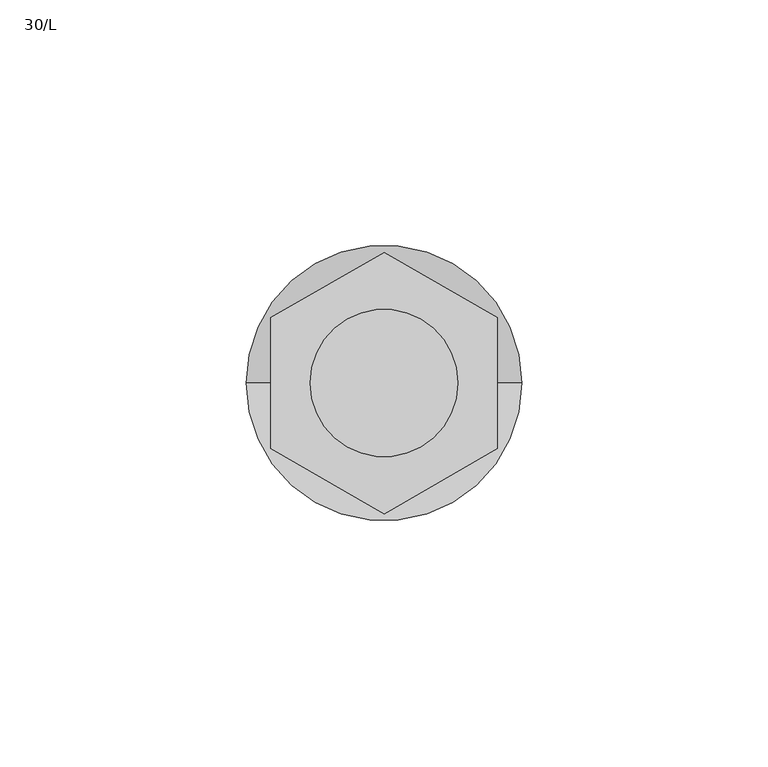
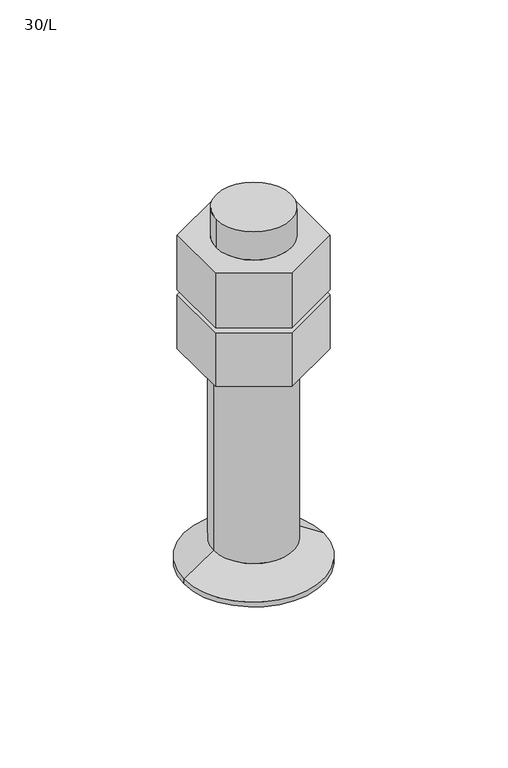
"""IFC4 building model written with IfcOpenShell, lengths in millimetres: fastener geometry, Bolt HPM-L : 30/L."""

from ifc_helpers import new_model, si_unit, frame, origin, origin_with_axes, place, context, project, spatial, polyline, circle_curve, source, transform, mapped, element, save
from ifc_brep_helpers import plane_surface, cylinder_surface, revolved_surface, advanced_brep


def fastener_30_l_a8502369(model_context):
    return source(origin(), model_context, "Body", "AdvancedBrep", [
        advanced_brep(
        [(-23.0, 13.2790562, 22.7), (-23.0, -13.2790562, 22.7), (0.0, -26.5581124, 22.7), (23.0, -13.2790562, 22.7), (23.0, 13.2790562, 22.7), (0.0, 26.5581124, 22.7), (15.0, 0.0, 22.7), (-15.0, 0.0, 22.7), (-23.0, 13.2790562, 0.0), (-23.0, -13.2790562, 0.0), (0.0, -26.5581124, 0.0), (23.0, -13.2790562, 0.0), (23.0, 13.2790562, 0.0), (0.0, 26.5581124, 0.0), (-15.0, 0.0, 60.0), (15.0, 0.0, 60.0), (15.0, 0.0, 25.0), (-15.0, 0.0, 25.0), (-15.0, 0.0, 48.0), (15.0, 0.0, 48.0), (-23.0, 13.2790562, 25.0), (0.0, 26.5581124, 25.0), (23.0, 13.2790562, 25.0), (23.0, -13.2790562, 25.0), (0.0, -26.5581124, 25.0), (-23.0, -13.2790562, 25.0), (-23.0, -13.2790562, 48.0), (-23.0, 13.2790562, 48.0), (0.0, -26.5581124, 48.0), (23.0, -13.2790562, 48.0), (23.0, 13.2790562, 48.0), (0.0, 26.5581124, 48.0), (-16.0, 0.0, 0.0), (-16.0, 0.0, -80.0), (16.0, 0.0, -80.0), (16.0, 0.0, 0.0), (-28.0, 0.0, -90.0), (28.0, 0.0, -90.0), (28.0, 0.0, -88.0), (-28.0, 0.0, -88.0)],
        [
            (0, 1),
            (1, 2),
            (2, 3),
            (3, 4),
            (4, 5),
            (5, 0),
            (6, 7, circle_curve(frame((0.0, 0.0, 22.7), z_axis=(0.0, 0.0, -1.0), x_axis=(1.0, 0.0, 0.0)), 15.0)),
            (7, 6, circle_curve(frame((0.0, 0.0, 22.7), z_axis=(0.0, 0.0, -1.0), x_axis=(1.0, 0.0, 0.0)), 15.0)),
            (0, 8),
            (8, 9),
            (9, 1),
            (9, 10),
            (10, 2),
            (10, 11),
            (11, 3),
            (11, 12),
            (12, 4),
            (12, 13),
            (13, 5),
            (13, 8),
            (14, 15, circle_curve(frame((0.0, 0.0, 60.0), z_axis=(0.0, 0.0, 1.0), x_axis=(1.0, 0.0, 0.0)), 15.0)),
            (15, 14, circle_curve(frame((0.0, 0.0, 60.0), z_axis=(0.0, 0.0, 1.0), x_axis=(1.0, 0.0, 0.0)), 15.0)),
            (6, 16),
            (16, 17, circle_curve(frame((0.0, 0.0, 25.0), z_axis=(0.0, 0.0, -1.0), x_axis=(1.0, 0.0, 0.0)), 15.0)),
            (17, 7),
            (14, 18),
            (18, 19, circle_curve(frame((0.0, 0.0, 48.0), z_axis=(0.0, 0.0, 1.0), x_axis=(1.0, 0.0, 0.0)), 15.0)),
            (19, 15),
            (17, 16, circle_curve(frame((0.0, 0.0, 25.0), z_axis=(0.0, 0.0, -1.0), x_axis=(1.0, 0.0, 0.0)), 15.0)),
            (19, 18, circle_curve(frame((0.0, 0.0, 48.0), z_axis=(0.0, 0.0, 1.0), x_axis=(1.0, 0.0, 0.0)), 15.0)),
            (20, 21),
            (21, 22),
            (22, 23),
            (23, 24),
            (24, 25),
            (25, 20),
            (26, 27),
            (27, 20),
            (25, 26),
            (28, 26),
            (24, 28),
            (29, 28),
            (23, 29),
            (30, 29),
            (22, 30),
            (31, 30),
            (21, 31),
            (27, 31),
            (32, 33),
            (33, 34, circle_curve(frame((0.0, 0.0, -80.0), z_axis=(0.0, 0.0, 1.0), x_axis=(1.0, 0.0, 0.0)), 16.0)),
            (34, 35),
            (35, 32, circle_curve(frame((0.0, 0.0, 0.0), z_axis=(0.0, 0.0, -1.0), x_axis=(1.0, 0.0, 0.0)), 16.0)),
            (32, 35, circle_curve(frame((0.0, 0.0, 0.0), z_axis=(0.0, 0.0, -1.0), x_axis=(1.0, 0.0, 0.0)), 16.0)),
            (34, 33, circle_curve(frame((0.0, 0.0, -80.0), z_axis=(0.0, 0.0, 1.0), x_axis=(1.0, 0.0, 0.0)), 16.0)),
            (36, 37, circle_curve(frame((0.0, 0.0, -90.0), z_axis=(0.0, 0.0, -1.0), x_axis=(1.0, 0.0, 0.0)), 28.0)),
            (37, 36, circle_curve(frame((0.0, 0.0, -90.0), z_axis=(0.0, 0.0, -1.0), x_axis=(1.0, 0.0, 0.0)), 28.0)),
            (37, 38),
            (38, 39, circle_curve(frame((0.0, 0.0, -88.0), z_axis=(0.0, 0.0, -1.0), x_axis=(1.0, 0.0, 0.0)), 28.0)),
            (39, 36),
            (39, 38, circle_curve(frame((0.0, 0.0, -88.0), z_axis=(0.0, 0.0, -1.0), x_axis=(1.0, 0.0, 0.0)), 28.0)),
            (33, 39),
            (38, 34),
        ],
        [
            plane_surface(frame((-23.0, 13.2790562, 22.7), z_axis=(0.0, 0.0, 1.0), x_axis=(0.0, -1.0, 0.0))),
            plane_surface(frame((-23.0, 13.2790562, 22.7), z_axis=(-1.0, 0.0, 0.0), x_axis=(0.0, 0.0, -1.0))),
            plane_surface(frame((-23.0, -13.2790562, 22.7), z_axis=(-0.4999999999999993, -0.8660254037844392, 0.0), x_axis=(0.0, 0.0, -1.0))),
            plane_surface(frame((0.0, -26.5581124, 22.7), z_axis=(0.5000000000000024, -0.8660254037844374, 0.0), x_axis=(0.0, 0.0, -1.0))),
            plane_surface(frame((23.0, -13.2790562, 22.7), z_axis=(1.0, 0.0, 0.0), x_axis=(0.0, 0.0, -1.0))),
            plane_surface(frame((23.0, 13.2790562, 22.7), z_axis=(0.4999999999999989, 0.8660254037844393, 0.0), x_axis=(0.0, 0.0, -1.0))),
            plane_surface(frame((0.0, 26.5581124, 22.7), z_axis=(-0.49999999999999895, 0.8660254037844393, 0.0), x_axis=(0.0, 0.0, -1.0))),
            plane_surface(frame((15.0, 0.0, 60.0), z_axis=(0.0, 0.0, 1.0), x_axis=(0.0, 1.0, 0.0))),
            cylinder_surface(origin_with_axes(), 15.0),
            plane_surface(frame((-23.0, 13.2790562, 25.0), z_axis=(0.0, 0.0, -1.0), x_axis=(0.0, 1.0, 0.0))),
            plane_surface(frame((-23.0, 13.2790562, 48.0), z_axis=(-1.0, 0.0, 0.0), x_axis=(0.0, 0.0, -1.0))),
            plane_surface(frame((-23.0, -13.2790562, 48.0), z_axis=(-0.4999999999999995, -0.866025403784439, 0.0), x_axis=(0.0, 0.0, -1.0))),
            plane_surface(frame((0.0, -26.5581124, 48.0), z_axis=(0.5000000000000024, -0.8660254037844373, 0.0), x_axis=(0.0, 0.0, -1.0))),
            plane_surface(frame((23.0, -13.2790562, 48.0), z_axis=(1.0, 0.0, 0.0), x_axis=(0.0, 0.0, -1.0))),
            plane_surface(frame((23.0, 13.2790562, 48.0), z_axis=(0.4999999999999991, 0.8660254037844393, 0.0), x_axis=(0.0, 0.0, -1.0))),
            plane_surface(frame((0.0, 26.5581124, 48.0), z_axis=(-0.49999999999999895, 0.8660254037844393, 0.0), x_axis=(0.0, 0.0, -1.0))),
            cylinder_surface(frame((0.0, 0.0, -80.0), z_axis=(0.0, 0.0, 1.0), x_axis=(1.0, 0.0, 0.0)), 16.0),
            plane_surface(frame((28.0, 0.0, -90.0), z_axis=(0.0, 0.0, -1.0), x_axis=(0.0, -1.0, 0.0))),
            cylinder_surface(frame((0.0, 0.0, -90.0), z_axis=(0.0, 0.0, 1.0), x_axis=(1.0, 0.0, 0.0)), 28.0),
            revolved_surface(polyline([(-16.00000002142857, 0.0, -80.0), (-28.0, 0.0, -88.0)]), (0.0, 0.0, -69.3333333), (0.0, 0.0, -1.0)),
            plane_surface(frame((-23.0, 13.2790562, 0.0), z_axis=(0.0, 0.0, -1.0), x_axis=(0.0, 1.0, 0.0))),
            plane_surface(frame((-23.0, 13.2790562, 48.0), z_axis=(0.0, 0.0, 1.0), x_axis=(0.0, -1.0, 0.0))),
        ],
        [
            (0, [[1, 2, 3, 4, 5, 6], [7, 8]]),
            (1, [[-1, 9, 10, 11]]),
            (2, [[-2, -11, 12, 13]]),
            (3, [[-3, -13, 14, 15]]),
            (4, [[-4, -15, 16, 17]]),
            (5, [[-5, -17, 18, 19]]),
            (6, [[-6, -19, 20, -9]]),
            (7, [[21, 22]]),
            (8, [[-7, 23, 24, 25]]),
            (8, [[-21, 26, 27, 28]]),
            (8, [[-8, -25, 29, -23]]),
            (8, [[-22, -28, 30, -26]]),
            (9, [[31, 32, 33, 34, 35, 36], [-24, -29]]),
            (10, [[37, 38, -36, 39]]),
            (11, [[40, -39, -35, 41]]),
            (12, [[42, -41, -34, 43]]),
            (13, [[44, -43, -33, 45]]),
            (14, [[46, -45, -32, 47]]),
            (15, [[48, -47, -31, -38]]),
            (16, [[49, 50, 51, 52]]),
            (16, [[-49, 53, -51, 54]]),
            (17, [[55, 56]]),
            (18, [[-56, 57, 58, 59]]),
            (18, [[-55, -59, 60, -57]]),
            (19, [[61, -58, 62, -50]]),
            (19, [[-61, -54, -62, -60]]),
            (20, [[-20, -18, -16, -14, -12, -10], [-52, -53]]),
            (21, [[-37, -40, -42, -44, -46, -48], [-27, -30]]),
        ],
    ),
    ])


if __name__ == "__main__":
    model = new_model("IFC4")
    model_context = context("Model", 3, world=origin())
    ifc_project = project(units=[si_unit("LENGTHUNIT", "METRE", prefix="MILLI")], contexts=[model_context])
    site = spatial("IfcSite", under=ifc_project)
    building = spatial("IfcBuilding", under=site)
    placement = place(None, origin())
    fastener_30_l_shape = fastener_30_l_a8502369(model_context)
    element("IfcFastener", 1, ObjectType="Bolt HPM-L : 30/L", at=placement, inside=building, context=model_context, shape_type="MappedRepresentation", body=[
        mapped(fastener_30_l_shape, transform((0.0, 0.0, 0.0), x_axis=(1.0, 0.0, 0.0), y_axis=(0.0, 1.0, 0.0), z_axis=(0.0, 0.0, 1.0))),
    ])
    save(model, "model.ifc")

# Revit data of these elements
# Type "Bolt HPM-L : 30/L"
#   Type Comments = "Mountingpart"
#   r3 = 15 mm
#   r2 = 28 mm
#   r1 = 16 mm
#   offset2 = 0 mm
#   l1 = 90 mm
#   Washer s = 8 mm
#   Washer Raduis2 = 32.5 mm
#   Washer Radius1 = 15.5 mm
#   Washer Diameter2 = 65 mm
#   Washer Diameter1 = 31 mm
#   T [instance default] = 45 mm
#   Offset1 [instance default] = 25 mm
#   Hexagonal nut m = 22.7 mm
#   l3 = 60 mm
#   l2 = 90 mm
#   hef = 80 mm
#   d3 = 30 mm
#   d1 = 32 mm
#   a = 60 mm
#   Hexagonal nut S1 = 23 mm
#   Hexagonal nut S = 46 mm
#   Material [instance default] = Metal - Steel - S355
#   Default Elevation = 0
# Element 1 (IfcFastener, "Bolt HPM-L : 30/L")
#   Materials on its faces: "Metal - Steel - S355"
# Materials
#   "Metal - Steel - S355": class "Steel", colour RGB 247 247 247, transparency 0, Cost = 0
